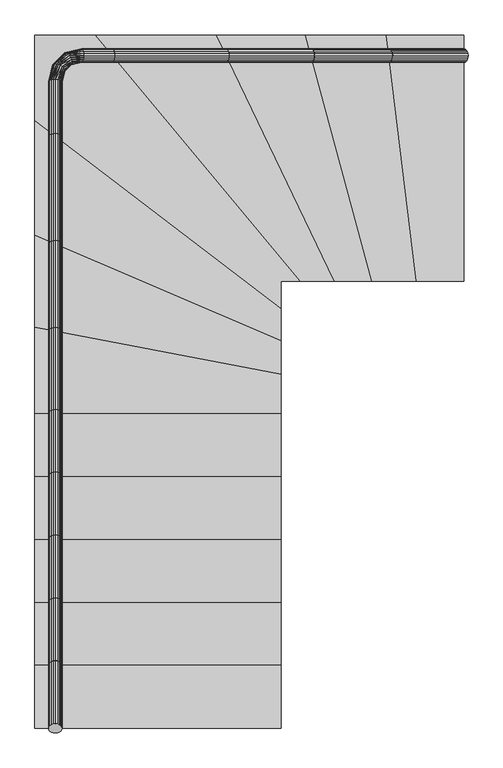
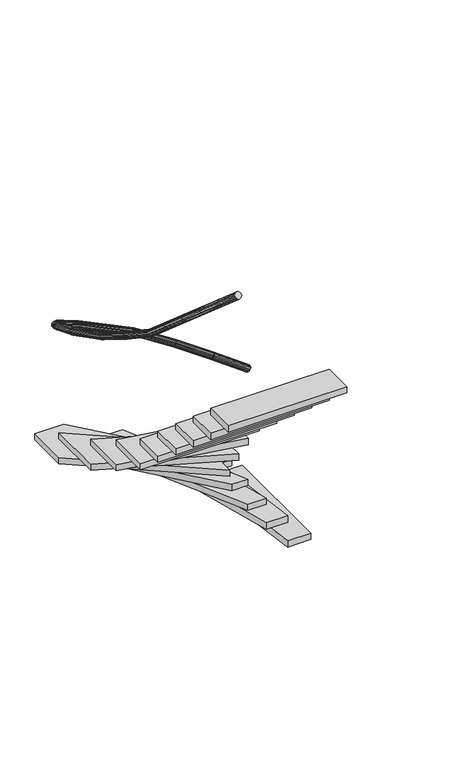
"""IFC4 building model written with IfcOpenShell, lengths in millimetres: stair geometry, 0_3d."""

from ifc_helpers import new_model, si_unit, frame, origin, origin_with_axes, place, context, project, spatial, polyline, outline, extrude, faceted_brep, source, transform, mapped, element, save


def stair_9af007b4(model_context):
    return source(origin(), model_context, "Body", "SolidModel", [
        extrude(outline(polyline([(1.2235871, -7.9923213), (0.0, 0.0), (1.2235871, 7.9923214), (4.7745751, 15.2022986), (10.3053687, 20.9241691), (17.2745751, 24.5978359), (25.0, 25.8636953), (32.7254249, 24.5978359), (39.6946313, 20.9241691), (45.2254249, 15.2022986), (48.7764129, 7.9923214), (50.0, 0.0), (48.7764129, -7.9923213), (45.2254249, -15.2022986), (39.6946313, -20.924169), (32.7254249, -24.5978359), (25.0, -25.8636953), (17.2745751, -24.5978359), (10.3053687, -20.924169), (4.7745751, -15.2022986), (1.2235871, -7.9923213)])), frame((50.0, 936.9712063, 2669.5592366), z_axis=(0.0, -0.7546055221634576, 0.6561787149248409), x_axis=(1.0, 0.0, 0.0)), (0.0, 0.0, 1.0), 304.7950131),
        extrude(outline(polyline([(970.0, 1651.5730429), (900.0, 1651.5730429), (900.0, 1551.5730429), (0.0, 2237.7659758), (0.0, 2551.5730429), (219.7566439, 2551.5730429), (970.0, 1651.5730429)])), frame((0.0, 0.0, 800.0), z_axis=(0.0, 0.0, 1.0), x_axis=(1.0, 0.0, 0.0)), (0.0, 0.0, 1.0), 50.0),
        extrude(outline(polyline([(1.2235871, -7.9923213), (0.0, 0.0), (1.2235871, 7.9923214), (4.7745751, 15.2022986), (10.3053687, 20.9241691), (17.2745751, 24.5978359), (25.0, 25.8636953), (32.7254249, 24.5978359), (39.6946313, 20.9241691), (45.2254249, 15.2022986), (48.7764129, 7.9923214), (50.0, 0.0), (48.7764129, -7.9923213), (45.2254249, -15.2022986), (39.6946313, -20.924169), (32.7254249, -24.5978359), (25.0, -25.8636953), (17.2745751, -24.5978359), (10.3053687, -20.924169), (4.7745751, -15.2022986), (1.2235871, -7.9923213)])), frame((50.0, 706.9712063, 2869.5592366), z_axis=(0.0, -0.7546055221634843, 0.6561787149248102), x_axis=(1.0, 0.0, 0.0)), (0.0, 0.0, 1.0), 304.7950131),
        extrude(outline(polyline([(1093.3486159, 1651.5730429), (970.0, 1651.5730429), (219.7566439, 2551.5730429), (662.4236343, 2551.5730429), (1093.3486159, 1651.5730429)])), frame((0.0, 0.0, 600.0), z_axis=(0.0, 0.0, 1.0), x_axis=(1.0, 0.0, 0.0)), (0.0, 0.0, 1.0), 50.0),
        faceted_brep([(51.2235871, 2177.2875031, 1862.2686626), (50.0, 2180.5832314, 1869.5592366), (51.2235871, 2183.8789598, 1876.8498106), (54.7745751, 2186.8520793, 1883.4267324), (60.3053687, 2189.2115603, 1888.6462072), (67.2745751, 2190.7264404, 1891.9973162), (75.0, 2191.2484324, 1893.1520297), (82.7254249, 2190.7264404, 1891.9973162), (89.6946313, 2189.2115603, 1888.6462072), (95.2254249, 2186.8520793, 1883.4267324), (98.7764129, 2183.8789598, 1876.8498106), (100.0, 2180.5832314, 1869.5592366), (98.7764129, 2177.2875031, 1862.2686626), (95.2254249, 2174.3143835, 1855.6917408), (89.6946313, 2171.9549025, 1850.4722661), (82.7254249, 2170.4400225, 1847.121157), (75.0, 2169.9180304, 1845.9664435), (67.2745751, 2170.4400225, 1847.121157), (60.3053687, 2171.9549025, 1850.4722661), (54.7745751, 2174.3143835, 1855.6917408), (51.2235871, 1791.6314427, 2076.5199053), (50.0, 1787.6876226, 2069.5592366), (51.2235871, 1783.7438024, 2062.5985679), (54.7745751, 1780.1860309, 2056.319258), (60.3053687, 1777.3625674, 2051.3359694), (67.2745751, 1775.5497922, 2048.1365012), (75.0, 1774.9251525, 2047.0340396), (82.7254249, 1775.5497922, 2048.1365012), (89.6946313, 1777.3625674, 2051.3359694), (95.2254249, 1780.1860309, 2056.319258), (98.7764129, 1783.7438024, 2062.5985679), (100.0, 1787.6876226, 2069.5592366), (98.7764129, 1791.6314427, 2076.5199053), (95.2254249, 1795.1892143, 2082.7992152), (89.6946313, 1798.0126778, 2087.7825038), (82.7254249, 1799.8254529, 2090.981972), (75.0, 1800.4500927, 2092.0844336), (67.2745751, 1799.8254529, 2090.981972), (60.3053687, 1798.0126778, 2087.7825038), (54.7745751, 1795.1892143, 2082.7992152)], [[[0, 1, 2, 3, 4, 5, 6, 7, 8, 9, 10, 11, 12, 13, 14, 15, 16, 17, 18, 19]], [[20, 21, 22, 23, 24, 25, 26, 27, 28, 29, 30, 31, 32, 33, 34, 35, 36, 37, 38, 39]], [[2, 1, 21, 20]], [[3, 2, 20, 39]], [[4, 3, 39, 38]], [[5, 4, 38, 37]], [[6, 5, 37, 36]], [[7, 6, 36, 35]], [[8, 7, 35, 34]], [[9, 8, 34, 33]], [[10, 9, 33, 32]], [[11, 10, 32, 31]], [[12, 11, 31, 30]], [[13, 12, 30, 29]], [[14, 13, 29, 28]], [[15, 14, 28, 27]], [[16, 15, 27, 26]], [[17, 16, 26, 25]], [[18, 17, 25, 24]], [[19, 18, 24, 23]], [[0, 19, 23, 22]], [[1, 0, 22, 21]]]),
        faceted_brep([(279.0658693, 2500.3494558, 1662.2350128), (282.2769235, 2501.5730429, 1669.5592366), (285.4879778, 2500.3494558, 1676.8834604), (288.3847117, 2496.7984678, 1683.4907382), (290.6835727, 2491.2676742, 1688.7343035), (292.1595323, 2484.2984678, 1692.1008796), (292.6681133, 2476.5730429, 1693.2609227), (292.1595323, 2468.8476181, 1692.1008796), (290.6835727, 2461.8784116, 1688.7343035), (288.3847117, 2456.3476181, 1683.4907382), (285.4879778, 2452.79663, 1676.8834604), (282.2769235, 2451.5730429, 1669.5592366), (279.0658693, 2452.79663, 1662.2350128), (276.1691354, 2456.3476181, 1655.627735), (273.8702744, 2461.8784116, 1650.3841697), (272.3943148, 2468.8476181, 1647.0175936), (271.8857337, 2476.5730429, 1645.8575505), (272.3943148, 2484.2984678, 1647.0175936), (273.8702744, 2491.2676742, 1650.3841697), (276.1691354, 2496.7984678, 1655.627735), (51.2235871, 2183.8789598, 1876.8498106), (50.0, 2180.5832314, 1869.5592366), (51.2235871, 2177.2875031, 1862.2686626), (54.7745751, 2174.3143835, 1855.6917408), (60.3053687, 2171.9549025, 1850.4722661), (67.2745751, 2170.4400225, 1847.121157), (75.0, 2169.9180304, 1845.9664435), (82.7254249, 2170.4400225, 1847.121157), (89.6946313, 2171.9549025, 1850.4722661), (95.2254249, 2174.3143835, 1855.6917408), (98.7764129, 2177.2875031, 1862.2686626), (100.0, 2180.5832314, 1869.5592366), (98.7764129, 2183.8789598, 1876.8498106), (95.2254249, 2186.8520793, 1883.4267324), (89.6946313, 2189.2115603, 1888.6462072), (82.7254249, 2190.7264404, 1891.9973162), (75.0, 2191.2484324, 1893.1520297), (67.2745751, 2190.7264404, 1891.9973162), (60.3053687, 2189.2115603, 1888.6462072), (54.7745751, 2186.8520793, 1883.4267324), (171.1411888, 2501.5730429, 1713.724975), (174.0928304, 2500.3494558, 1721.1522903), (176.7555448, 2496.7984678, 1727.8525682), (178.8686869, 2491.2676742, 1733.1699389), (180.2254077, 2484.2984678, 1736.583901), (180.6929018, 2476.5730429, 1737.7602722), (180.2254077, 2468.8476181, 1736.583901), (178.8686869, 2461.8784116, 1733.1699389), (176.7555448, 2456.3476181, 1727.8525682), (174.0928304, 2452.79663, 1721.1522903), (171.1411888, 2451.5730429, 1713.724975), (168.1895471, 2452.79663, 1706.2976597), (165.5268327, 2456.3476181, 1699.5973818), (163.4136906, 2461.8784116, 1694.2800111), (162.0569698, 2468.8476181, 1690.866049), (161.5894757, 2476.5730429, 1689.6896778), (162.0569698, 2484.2984678, 1690.866049), (163.4136906, 2491.2676742, 1694.2800111), (165.5268327, 2496.7984678, 1699.5973818), (168.1895471, 2500.3494558, 1706.2976597), (108.4388924, 2486.457503, 1738.6559048), (112.3547346, 2487.2072116, 1745.6899991), (117.06286, 2485.7372245, 1752.0355473), (122.1024044, 2482.1914344, 1757.0714029), (126.9800623, 2476.9169277, 1760.3046212), (131.2183743, 2470.43001, 1761.4187123), (134.4024651, 2463.365666, 1760.3046212), (136.2206536, 2456.4154029, 1757.0714029), (136.4949629, 2450.2595609, 1752.0355473), (135.1985416, 2445.5007167, 1745.6899991), (132.4582926, 2442.604699, 1738.6559048), (128.5424504, 2441.8549904, 1731.6218104), (123.834325, 2443.3249774, 1725.2762623), (118.7947805, 2446.8707676, 1720.2404067), (113.9171227, 2452.1452743, 1717.0071884), (109.6788106, 2458.632192, 1715.8930973), (106.4947198, 2465.696536, 1717.0071884), (104.6765313, 2472.6467991, 1720.2404067), (104.402222, 2478.8026411, 1725.2762623), (105.6986433, 2483.5614853, 1731.6218104), (65.11554, 2443.1341506, 1765.2077495), (68.0115576, 2445.8743996, 1772.2418439), (72.7704018, 2447.1708209, 1778.5873921), (78.9262439, 2446.8965116, 1783.6232476), (85.876507, 2445.0783231, 1786.8564659), (92.940851, 2441.8942323, 1787.970557), (99.4277686, 2437.6559202, 1786.8564659), (104.7022753, 2432.7782624, 1783.6232476), (108.2480655, 2427.7387179, 1778.5873921), (109.7180525, 2423.0305925, 1772.2418439), (108.9683439, 2419.1147504, 1765.2077495), (106.0723263, 2416.3745013, 1758.1736552), (101.313482, 2415.07808, 1751.828107), (95.15764, 2415.3523893, 1746.7922515), (88.2073769, 2417.1705778, 1743.5590332), (81.1430329, 2420.3546686, 1742.4449421), (74.6561152, 2424.5929807, 1743.5590332), (69.3816086, 2429.4706385, 1746.7922515), (65.8358184, 2434.510183, 1751.828107), (64.3658313, 2439.2183084, 1758.1736552), (50.0, 2380.4318542, 1790.1386793), (51.2235871, 2383.3834958, 1797.5659946), (54.7745751, 2386.0462102, 1804.2662726), (60.3053687, 2388.1593524, 1809.5836432), (67.2745751, 2389.5160731, 1812.9976054), (75.0, 2389.9835672, 1814.1739765), (82.7254249, 2389.5160731, 1812.9976054), (89.6946313, 2388.1593524, 1809.5836432), (95.2254249, 2386.0462102, 1804.2662726), (98.7764129, 2383.3834958, 1797.5659946), (100.0, 2380.4318542, 1790.1386793), (98.7764129, 2377.4802125, 1782.711364), (95.2254249, 2374.8174981, 1776.0110861), (89.6946313, 2372.704356, 1770.6937155), (82.7254249, 2371.3476352, 1767.2797533), (75.0, 2370.8801411, 1766.1033822), (67.2745751, 2371.3476352, 1767.2797533), (60.3053687, 2372.704356, 1770.6937155), (54.7745751, 2374.8174981, 1776.0110861), (51.2235871, 2377.4802125, 1782.711364)], [[[0, 1, 2, 3, 4, 5, 6, 7, 8, 9, 10, 11, 12, 13, 14, 15, 16, 17, 18, 19]], [[20, 21, 22, 23, 24, 25, 26, 27, 28, 29, 30, 31, 32, 33, 34, 35, 36, 37, 38, 39]], [[2, 1, 40, 41]], [[3, 2, 41, 42]], [[4, 3, 42, 43]], [[5, 4, 43, 44]], [[6, 5, 44, 45]], [[7, 6, 45, 46]], [[8, 7, 46, 47]], [[9, 8, 47, 48]], [[10, 9, 48, 49]], [[11, 10, 49, 50]], [[12, 11, 50, 51]], [[13, 12, 51, 52]], [[14, 13, 52, 53]], [[15, 14, 53, 54]], [[16, 15, 54, 55]], [[17, 16, 55, 56]], [[18, 17, 56, 57]], [[19, 18, 57, 58]], [[0, 19, 58, 59]], [[1, 0, 59, 40]], [[41, 40, 60]], [[61, 41, 60]], [[42, 41, 61]], [[62, 42, 61]], [[43, 42, 62]], [[63, 43, 62]], [[44, 43, 63]], [[64, 44, 63]], [[45, 44, 64]], [[65, 45, 64]], [[46, 45, 65]], [[66, 46, 65]], [[47, 46, 66]], [[67, 47, 66]], [[48, 47, 67]], [[68, 48, 67]], [[49, 48, 68]], [[69, 49, 68]], [[50, 49, 69]], [[70, 50, 69]], [[51, 50, 70]], [[71, 51, 70]], [[52, 51, 71]], [[72, 52, 71]], [[53, 52, 72]], [[73, 53, 72]], [[54, 53, 73]], [[74, 54, 73]], [[55, 54, 74]], [[75, 55, 74]], [[56, 55, 75]], [[76, 56, 75]], [[57, 56, 76]], [[77, 57, 76]], [[58, 57, 77]], [[78, 58, 77]], [[59, 58, 78]], [[79, 59, 78]], [[40, 59, 79]], [[60, 40, 79]], [[61, 60, 80]], [[81, 61, 80]], [[62, 61, 81]], [[82, 62, 81]], [[63, 62, 82]], [[83, 63, 82]], [[64, 63, 83]], [[84, 64, 83]], [[65, 64, 84]], [[85, 65, 84]], [[66, 65, 85]], [[86, 66, 85]], [[67, 66, 86]], [[87, 67, 86]], [[68, 67, 87]], [[88, 68, 87]], [[69, 68, 88]], [[89, 69, 88]], [[70, 69, 89]], [[90, 70, 89]], [[71, 70, 90]], [[91, 71, 90]], [[72, 71, 91]], [[92, 72, 91]], [[73, 72, 92]], [[93, 73, 92]], [[74, 73, 93]], [[94, 74, 93]], [[75, 74, 94]], [[95, 75, 94]], [[76, 75, 95]], [[96, 76, 95]], [[77, 76, 96]], [[97, 77, 96]], [[78, 77, 97]], [[98, 78, 97]], [[79, 78, 98]], [[99, 79, 98]], [[60, 79, 99]], [[80, 60, 99]], [[81, 80, 100]], [[101, 81, 100]], [[82, 81, 101]], [[102, 82, 101]], [[83, 82, 102]], [[103, 83, 102]], [[84, 83, 103]], [[104, 84, 103]], [[85, 84, 104]], [[105, 85, 104]], [[86, 85, 105]], [[106, 86, 105]], [[87, 86, 106]], [[107, 87, 106]], [[88, 87, 107]], [[108, 88, 107]], [[89, 88, 108]], [[109, 89, 108]], [[90, 89, 109]], [[110, 90, 109]], [[91, 90, 110]], [[111, 91, 110]], [[92, 91, 111]], [[112, 92, 111]], [[93, 92, 112]], [[113, 93, 112]], [[94, 93, 113]], [[114, 94, 113]], [[95, 94, 114]], [[115, 95, 114]], [[96, 95, 115]], [[116, 96, 115]], [[97, 96, 116]], [[117, 97, 116]], [[98, 97, 117]], [[118, 98, 117]], [[99, 98, 118]], [[119, 99, 118]], [[80, 99, 119]], [[100, 80, 119]], [[101, 100, 21, 20]], [[102, 101, 20, 39]], [[103, 102, 39, 38]], [[104, 103, 38, 37]], [[105, 104, 37, 36]], [[106, 105, 36, 35]], [[107, 106, 35, 34]], [[108, 107, 34, 33]], [[109, 108, 33, 32]], [[110, 109, 32, 31]], [[111, 110, 31, 30]], [[112, 111, 30, 29]], [[113, 112, 29, 28]], [[114, 113, 28, 27]], [[115, 114, 27, 26]], [[116, 115, 26, 25]], [[117, 116, 25, 24]], [[118, 117, 24, 23]], [[119, 118, 23, 22]], [[100, 119, 22, 21]]]),
        faceted_brep([(51.2235871, 1162.120888, 2463.1855148), (50.0, 1166.9712063, 2469.5592366), (51.2235871, 1171.8215247, 2475.9329585), (54.7745751, 1176.1970601, 2481.682776), (60.3053687, 1179.6695046, 2486.2458571), (67.2745751, 1181.8989513, 2489.1755354), (75.0, 1182.6671663, 2490.1850338), (82.7254249, 1181.8989513, 2489.1755354), (89.6946313, 1179.6695046, 2486.2458571), (95.2254249, 1176.1970601, 2481.682776), (98.7764129, 1171.8215247, 2475.9329585), (100.0, 1166.9712063, 2469.5592366), (98.7764129, 1162.120888, 2463.1855148), (95.2254249, 1157.7453526, 2457.4356972), (89.6946313, 1154.272908, 2452.8726162), (82.7254249, 1152.0434614, 2449.9429378), (75.0, 1151.2752464, 2448.9334394), (67.2745751, 1152.0434614, 2449.9429378), (60.3053687, 1154.272908, 2452.8726162), (54.7745751, 1157.7453526, 2457.4356972), (51.2235871, 942.2155975, 2675.5902865), (50.0, 936.9712063, 2669.5592366), (51.2235871, 931.7268152, 2663.5281868), (54.7745751, 926.9957815, 2658.0874981), (60.3053687, 923.241212, 2653.7697431), (67.2745751, 920.83063, 2650.9975738), (75.0, 920.0, 2650.0423493), (82.7254249, 920.83063, 2650.9975738), (89.6946313, 923.241212, 2653.7697431), (95.2254249, 926.9957815, 2658.0874981), (98.7764129, 931.7268152, 2663.5281868), (100.0, 936.9712063, 2669.5592366), (98.7764129, 942.2155975, 2675.5902865), (95.2254249, 946.9466311, 2681.0309751), (89.6946313, 950.7012007, 2685.3487301), (82.7254249, 953.1117827, 2688.1208994), (75.0, 953.9424127, 2689.0761239), (67.2745751, 953.1117827, 2688.1208994), (60.3053687, 950.7012007, 2685.3487301), (54.7745751, 946.9466311, 2681.0309751)], [[[0, 1, 2, 3, 4, 5, 6, 7, 8, 9, 10, 11, 12, 13, 14, 15, 16, 17, 18, 19]], [[20, 21, 22, 23, 24, 25, 26, 27, 28, 29, 30, 31, 32, 33, 34, 35, 36, 37, 38, 39]], [[2, 1, 21, 20]], [[3, 2, 20, 39]], [[4, 3, 39, 38]], [[5, 4, 38, 37]], [[6, 5, 37, 36]], [[7, 6, 36, 35]], [[8, 7, 35, 34]], [[9, 8, 34, 33]], [[10, 9, 33, 32]], [[11, 10, 32, 31]], [[12, 11, 31, 30]], [[13, 12, 30, 29]], [[14, 13, 29, 28]], [[15, 14, 28, 27]], [[16, 15, 27, 26]], [[17, 16, 26, 25]], [[18, 17, 25, 24]], [[19, 18, 24, 23]], [[0, 19, 23, 22]], [[1, 0, 22, 21]]]),
        extrude(outline(polyline([(900.0, 936.9712063), (900.0, 706.9712063), (0.0, 706.9712063), (0.0, 936.9712063), (900.0, 936.9712063)])), frame((0.0, 0.0, 1800.0), z_axis=(0.0, 0.0, 1.0), x_axis=(1.0, 0.0, 0.0)), (0.0, 0.0, 1.0), 50.0),
        extrude(outline(polyline([(900.0, 1310.8135078), (900.0, 1166.9712063), (0.0, 1166.9712063), (0.0, 1483.1289049), (900.0, 1310.8135078)])), frame((0.0, 0.0, 1400.0), z_axis=(0.0, 0.0, 1.0), x_axis=(1.0, 0.0, 0.0)), (0.0, 0.0, 1.0), 50.0),
        extrude(outline(polyline([(900.0, 1434.6945611), (900.0, 1310.8135078), (0.0, 1483.1289049), (0.0, 1819.7779009), (900.0, 1434.6945611)])), frame((0.0, 0.0, 1200.0), z_axis=(0.0, 0.0, 1.0), x_axis=(1.0, 0.0, 0.0)), (0.0, 0.0, 1.0), 50.0),
        faceted_brep([(1565.3069331, 2500.3494558, 863.0898994), (1570.0, 2501.5730429, 869.5592366), (1574.6930669, 2500.3494558, 876.0285738), (1578.9267437, 2496.7984678, 881.8646473), (1582.2866086, 2491.2676742, 886.4961814), (1584.4437746, 2484.2984678, 889.4698093), (1585.1870834, 2476.5730429, 890.4944517), (1584.4437746, 2468.8476181, 889.4698093), (1582.2866086, 2461.8784116, 886.4961814), (1578.9267437, 2456.3476181, 881.8646473), (1574.6930669, 2452.79663, 876.0285738), (1570.0, 2451.5730429, 869.5592366), (1565.3069331, 2452.79663, 863.0898994), (1561.0732563, 2456.3476181, 857.2538259), (1557.7133914, 2461.8784116, 852.6222918), (1555.5562254, 2468.8476181, 849.6486639), (1554.8129166, 2476.5730429, 848.6240215), (1555.5562254, 2484.2984678, 849.6486639), (1557.7133914, 2491.2676742, 852.6222918), (1561.0732563, 2496.7984678, 857.2538259), (1298.9424936, 2500.3494558, 1076.0669753), (1294.3023627, 2501.5730429, 1069.5592366), (1289.6622317, 2500.3494558, 1063.0514979), (1285.4763091, 2496.7984678, 1057.1807821), (1282.1543421, 2491.2676742, 1052.5217556), (1280.021508, 2484.2984678, 1049.5304765), (1279.2865835, 2476.5730429, 1048.4997519), (1280.021508, 2468.8476181, 1049.5304765), (1282.1543421, 2461.8784116, 1052.5217556), (1285.4763091, 2456.3476181, 1057.1807821), (1289.6622317, 2452.79663, 1063.0514979), (1294.3023627, 2451.5730429, 1069.5592366), (1298.9424936, 2452.79663, 1076.0669753), (1303.1284163, 2456.3476181, 1081.9376911), (1306.4503833, 2461.8784116, 1086.5967176), (1308.5832174, 2468.8476181, 1089.5879968), (1309.3181419, 2476.5730429, 1090.6187213), (1308.5832174, 2484.2984678, 1089.5879968), (1306.4503833, 2491.2676742, 1086.5967176), (1303.1284163, 2496.7984678, 1081.9376911)], [[[0, 1, 2, 3, 4, 5, 6, 7, 8, 9, 10, 11, 12, 13, 14, 15, 16, 17, 18, 19]], [[20, 21, 22, 23, 24, 25, 26, 27, 28, 29, 30, 31, 32, 33, 34, 35, 36, 37, 38, 39]], [[2, 1, 21, 20]], [[3, 2, 20, 39]], [[4, 3, 39, 38]], [[5, 4, 38, 37]], [[6, 5, 37, 36]], [[7, 6, 36, 35]], [[8, 7, 35, 34]], [[9, 8, 34, 33]], [[10, 9, 33, 32]], [[11, 10, 32, 31]], [[12, 11, 31, 30]], [[13, 12, 30, 29]], [[14, 13, 29, 28]], [[15, 14, 28, 27]], [[16, 15, 27, 26]], [[17, 16, 26, 25]], [[18, 17, 25, 24]], [[19, 18, 24, 23]], [[0, 19, 23, 22]], [[1, 0, 22, 21]]]),
        extrude(outline(polyline([(1.2235871, -7.9923213), (0.0, 0.0), (1.2235871, 7.9923214), (4.7745751, 15.2022986), (10.3053687, 20.9241691), (17.2745751, 24.5978359), (25.0, 25.8636953), (32.7254249, 24.5978359), (39.6946313, 20.9241691), (45.2254249, 15.2022986), (48.7764129, 7.9923214), (50.0, 0.0), (48.7764129, -7.9923213), (45.2254249, -15.2022986), (39.6946313, -20.924169), (32.7254249, -24.5978359), (25.0, -25.8636953), (17.2745751, -24.5978359), (10.3053687, -20.924169), (4.7745751, -15.2022986), (1.2235871, -7.9923213)])), frame((50.0, 476.9712063, 3069.5592366), z_axis=(0.0, -0.754605522163458, 0.6561787149248404), x_axis=(1.0, 0.0, 0.0)), (0.0, 0.0, 1.0), 304.7950131),
        faceted_brep([(51.2235871, 1464.4379829, 2262.8415677), (50.0, 1468.7692885, 2269.5592366), (51.2235871, 1473.100594, 2276.2769055), (54.7745751, 1477.0079212, 2282.3370022), (60.3053687, 1480.1087936, 2287.1463221), (67.2745751, 1482.0996763, 2290.2340956), (75.0, 1482.7856877, 2291.2980698), (82.7254249, 1482.0996763, 2290.2340956), (89.6946313, 1480.1087936, 2287.1463221), (95.2254249, 1477.0079212, 2282.3370022), (98.7764129, 1473.100594, 2276.2769055), (100.0, 1468.7692885, 2269.5592366), (98.7764129, 1464.4379829, 2262.8415677), (95.2254249, 1460.5306557, 2256.781471), (89.6946313, 1457.4297833, 2251.9721511), (82.7254249, 1455.4389007, 2248.8843776), (75.0, 1454.7528893, 2247.8204034), (67.2745751, 1455.4389007, 2248.8843776), (60.3053687, 1457.4297833, 2251.9721511), (54.7745751, 1460.5306557, 2256.781471), (51.2235871, 1171.8215247, 2475.9329585), (50.0, 1166.9712063, 2469.5592366), (51.2235871, 1162.120888, 2463.1855148), (54.7745751, 1157.7453526, 2457.4356972), (60.3053687, 1154.272908, 2452.8726162), (67.2745751, 1152.0434614, 2449.9429378), (75.0, 1151.2752464, 2448.9334394), (82.7254249, 1152.0434614, 2449.9429378), (89.6946313, 1154.272908, 2452.8726162), (95.2254249, 1157.7453526, 2457.4356972), (98.7764129, 1162.120888, 2463.1855148), (100.0, 1166.9712063, 2469.5592366), (98.7764129, 1171.8215247, 2475.9329585), (95.2254249, 1176.1970601, 2481.682776), (89.6946313, 1179.6695046, 2486.2458571), (82.7254249, 1181.8989513, 2489.1755354), (75.0, 1182.6671663, 2490.1850338), (67.2745751, 1181.8989513, 2489.1755354), (60.3053687, 1179.6695046, 2486.2458571), (54.7745751, 1176.1970601, 2481.682776)], [[[0, 1, 2, 3, 4, 5, 6, 7, 8, 9, 10, 11, 12, 13, 14, 15, 16, 17, 18, 19]], [[20, 21, 22, 23, 24, 25, 26, 27, 28, 29, 30, 31, 32, 33, 34, 35, 36, 37, 38, 39]], [[2, 1, 21, 20]], [[3, 2, 20, 39]], [[4, 3, 39, 38]], [[5, 4, 38, 37]], [[6, 5, 37, 36]], [[7, 6, 36, 35]], [[8, 7, 35, 34]], [[9, 8, 34, 33]], [[10, 9, 33, 32]], [[11, 10, 32, 31]], [[12, 11, 31, 30]], [[13, 12, 30, 29]], [[14, 13, 29, 28]], [[15, 14, 28, 27]], [[16, 15, 27, 26]], [[17, 16, 26, 25]], [[18, 17, 25, 24]], [[19, 18, 24, 23]], [[0, 19, 23, 22]], [[1, 0, 22, 21]]]),
        extrude(outline(polyline([(900.0, 1551.5730429), (900.0, 1434.6945611), (0.0, 1819.7779009), (0.0, 2237.7659758), (900.0, 1551.5730429)])), frame((0.0, 0.0, 1000.0), z_axis=(0.0, 0.0, 1.0), x_axis=(1.0, 0.0, 0.0)), (0.0, 0.0, 1.0), 50.0),
        extrude(outline(polyline([(1231.3290941, 1651.5730429), (1093.3486159, 1651.5730429), (662.4236343, 2551.5730429), (988.6709059, 2551.5730429), (1231.3290941, 1651.5730429)])), frame((0.0, 0.0, 400.0), z_axis=(0.0, 0.0, 1.0), x_axis=(1.0, 0.0, 0.0)), (0.0, 0.0, 1.0), 50.0),
        faceted_brep([(694.4240305, 2500.3494558, 1462.5710073), (698.3340494, 2501.5730429, 1469.5592366), (702.2440682, 2500.3494558, 1476.5474659), (705.7713472, 2496.7984678, 1482.8516386), (708.5706116, 2491.2676742, 1487.8546583), (710.36785, 2484.2984678, 1491.0667948), (710.9871362, 2476.5730429, 1492.1736216), (710.36785, 2468.8476181, 1491.0667948), (708.5706116, 2461.8784116, 1487.8546583), (705.7713472, 2456.3476181, 1482.8516386), (702.2440682, 2452.79663, 1476.5474659), (698.3340494, 2451.5730429, 1469.5592366), (694.4240305, 2452.79663, 1462.5710073), (690.8967516, 2456.3476181, 1456.2668346), (688.0974871, 2461.8784116, 1451.2638149), (686.3002487, 2468.8476181, 1448.0516784), (685.6809626, 2476.5730429, 1446.9448517), (686.3002487, 2484.2984678, 1448.0516784), (688.0974871, 2491.2676742, 1451.2638149), (690.8967516, 2496.7984678, 1456.2668346), (285.4879778, 2500.3494558, 1676.8834604), (282.2769235, 2501.5730429, 1669.5592366), (279.0658693, 2500.3494558, 1662.2350128), (276.1691354, 2496.7984678, 1655.627735), (273.8702744, 2491.2676742, 1650.3841697), (272.3943148, 2484.2984678, 1647.0175936), (271.8857337, 2476.5730429, 1645.8575505), (272.3943148, 2468.8476181, 1647.0175936), (273.8702744, 2461.8784116, 1650.3841697), (276.1691354, 2456.3476181, 1655.627735), (279.0658693, 2452.79663, 1662.2350128), (282.2769235, 2451.5730429, 1669.5592366), (285.4879778, 2452.79663, 1676.8834604), (288.3847117, 2456.3476181, 1683.4907382), (290.6835727, 2461.8784116, 1688.7343035), (292.1595323, 2468.8476181, 1692.1008796), (292.6681133, 2476.5730429, 1693.2609227), (292.1595323, 2484.2984678, 1692.1008796), (290.6835727, 2491.2676742, 1688.7343035), (288.3847117, 2496.7984678, 1683.4907382)], [[[0, 1, 2, 3, 4, 5, 6, 7, 8, 9, 10, 11, 12, 13, 14, 15, 16, 17, 18, 19]], [[20, 21, 22, 23, 24, 25, 26, 27, 28, 29, 30, 31, 32, 33, 34, 35, 36, 37, 38, 39]], [[2, 1, 21, 20]], [[3, 2, 20, 39]], [[4, 3, 39, 38]], [[5, 4, 38, 37]], [[6, 5, 37, 36]], [[7, 6, 36, 35]], [[8, 7, 35, 34]], [[9, 8, 34, 33]], [[10, 9, 33, 32]], [[11, 10, 32, 31]], [[12, 11, 31, 30]], [[13, 12, 30, 29]], [[14, 13, 29, 28]], [[15, 14, 28, 27]], [[16, 15, 27, 26]], [[17, 16, 26, 25]], [[18, 17, 25, 24]], [[19, 18, 24, 23]], [[0, 19, 23, 22]], [[1, 0, 22, 21]]]),
        extrude(outline(polyline([(900.0, 1166.9712063), (900.0, 936.9712063), (0.0, 936.9712063), (0.0, 1166.9712063), (900.0, 1166.9712063)])), frame((0.0, 0.0, 1600.0), z_axis=(0.0, 0.0, 1.0), x_axis=(1.0, 0.0, 0.0)), (0.0, 0.0, 1.0), 50.0),
        faceted_brep([(1289.6622317, 2500.3494558, 1063.0514979), (1294.3023627, 2501.5730429, 1069.5592366), (1298.9424936, 2500.3494558, 1076.0669753), (1303.1284163, 2496.7984678, 1081.9376911), (1306.4503833, 2491.2676742, 1086.5967176), (1308.5832174, 2484.2984678, 1089.5879968), (1309.3181419, 2476.5730429, 1090.6187213), (1308.5832174, 2468.8476181, 1089.5879968), (1306.4503833, 2461.8784116, 1086.5967176), (1303.1284163, 2456.3476181, 1081.9376911), (1298.9424936, 2452.79663, 1076.0669753), (1294.3023627, 2451.5730429, 1069.5592366), (1289.6622317, 2452.79663, 1063.0514979), (1285.4763091, 2456.3476181, 1057.1807821), (1282.1543421, 2461.8784116, 1052.5217556), (1280.021508, 2468.8476181, 1049.5304765), (1279.2865835, 2476.5730429, 1048.4997519), (1280.021508, 2484.2984678, 1049.5304765), (1282.1543421, 2491.2676742, 1052.5217556), (1285.4763091, 2496.7984678, 1057.1807821), (1013.3510842, 2500.3494558, 1276.1941386), (1008.8924216, 2501.5730429, 1269.5592366), (1004.433759, 2500.3494558, 1262.9243346), (1000.4115414, 2496.7984678, 1256.9389031), (997.2194914, 2491.2676742, 1252.1888377), (995.1700692, 2484.2984678, 1249.139108), (994.4638864, 2476.5730429, 1248.0882427), (995.1700692, 2468.8476181, 1249.139108), (997.2194914, 2461.8784116, 1252.1888377), (1000.4115414, 2456.3476181, 1256.9389031), (1004.433759, 2452.79663, 1262.9243346), (1008.8924216, 2451.5730429, 1269.5592366), (1013.3510842, 2452.79663, 1276.1941386), (1017.3733018, 2456.3476181, 1282.1795702), (1020.5653518, 2461.8784116, 1286.9296355), (1022.614774, 2468.8476181, 1289.9793652), (1023.3209568, 2476.5730429, 1291.0302305), (1022.614774, 2484.2984678, 1289.9793652), (1020.5653518, 2491.2676742, 1286.9296355), (1017.3733018, 2496.7984678, 1282.1795702)], [[[0, 1, 2, 3, 4, 5, 6, 7, 8, 9, 10, 11, 12, 13, 14, 15, 16, 17, 18, 19]], [[20, 21, 22, 23, 24, 25, 26, 27, 28, 29, 30, 31, 32, 33, 34, 35, 36, 37, 38, 39]], [[2, 1, 21, 20]], [[3, 2, 20, 39]], [[4, 3, 39, 38]], [[5, 4, 38, 37]], [[6, 5, 37, 36]], [[7, 6, 36, 35]], [[8, 7, 35, 34]], [[9, 8, 34, 33]], [[10, 9, 33, 32]], [[11, 10, 32, 31]], [[12, 11, 31, 30]], [[13, 12, 30, 29]], [[14, 13, 29, 28]], [[15, 14, 28, 27]], [[16, 15, 27, 26]], [[17, 16, 26, 25]], [[18, 17, 25, 24]], [[19, 18, 24, 23]], [[0, 19, 23, 22]], [[1, 0, 22, 21]]]),
        faceted_brep([(51.2235871, 1783.7438024, 2062.5985679), (50.0, 1787.6876226, 2069.5592366), (51.2235871, 1791.6314427, 2076.5199053), (54.7745751, 1795.1892143, 2082.7992152), (60.3053687, 1798.0126778, 2087.7825038), (67.2745751, 1799.8254529, 2090.981972), (75.0, 1800.4500927, 2092.0844336), (82.7254249, 1799.8254529, 2090.981972), (89.6946313, 1798.0126778, 2087.7825038), (95.2254249, 1795.1892143, 2082.7992152), (98.7764129, 1791.6314427, 2076.5199053), (100.0, 1787.6876226, 2069.5592366), (98.7764129, 1783.7438024, 2062.5985679), (95.2254249, 1780.1860309, 2056.319258), (89.6946313, 1777.3625674, 2051.3359694), (82.7254249, 1775.5497922, 2048.1365012), (75.0, 1774.9251525, 2047.0340396), (67.2745751, 1775.5497922, 2048.1365012), (60.3053687, 1777.3625674, 2051.3359694), (54.7745751, 1780.1860309, 2056.319258), (51.2235871, 1473.100594, 2276.2769055), (50.0, 1468.7692885, 2269.5592366), (51.2235871, 1464.4379829, 2262.8415677), (54.7745751, 1460.5306557, 2256.781471), (60.3053687, 1457.4297833, 2251.9721511), (67.2745751, 1455.4389007, 2248.8843776), (75.0, 1454.7528893, 2247.8204034), (82.7254249, 1455.4389007, 2248.8843776), (89.6946313, 1457.4297833, 2251.9721511), (95.2254249, 1460.5306557, 2256.781471), (98.7764129, 1464.4379829, 2262.8415677), (100.0, 1468.7692885, 2269.5592366), (98.7764129, 1473.100594, 2276.2769055), (95.2254249, 1477.0079212, 2282.3370022), (89.6946313, 1480.1087936, 2287.1463221), (82.7254249, 1482.0996763, 2290.2340956), (75.0, 1482.7856877, 2291.2980698), (67.2745751, 1482.0996763, 2290.2340956), (60.3053687, 1480.1087936, 2287.1463221), (54.7745751, 1477.0079212, 2282.3370022)], [[[0, 1, 2, 3, 4, 5, 6, 7, 8, 9, 10, 11, 12, 13, 14, 15, 16, 17, 18, 19]], [[20, 21, 22, 23, 24, 25, 26, 27, 28, 29, 30, 31, 32, 33, 34, 35, 36, 37, 38, 39]], [[2, 1, 21, 20]], [[3, 2, 20, 39]], [[4, 3, 39, 38]], [[5, 4, 38, 37]], [[6, 5, 37, 36]], [[7, 6, 36, 35]], [[8, 7, 35, 34]], [[9, 8, 34, 33]], [[10, 9, 33, 32]], [[11, 10, 32, 31]], [[12, 11, 31, 30]], [[13, 12, 30, 29]], [[14, 13, 29, 28]], [[15, 14, 28, 27]], [[16, 15, 27, 26]], [[17, 16, 26, 25]], [[18, 17, 25, 24]], [[19, 18, 24, 23]], [[0, 19, 23, 22]], [[1, 0, 22, 21]]]),
        extrude(outline(polyline([(1394.8371648, 1651.5730429), (1231.3290941, 1651.5730429), (988.6709059, 2551.5730429), (1285.1628352, 2551.5730429), (1394.8371648, 1651.5730429)])), frame((0.0, 0.0, 200.0), z_axis=(0.0, 0.0, 1.0), x_axis=(1.0, 0.0, 0.0)), (0.0, 0.0, 1.0), 50.0),
        extrude(outline(polyline([(1570.0, 1651.5730429), (1394.8371648, 1651.5730429), (1285.1628352, 2551.5730429), (1570.0, 2551.5730429), (1570.0, 1651.5730429)])), origin_with_axes(), (0.0, 0.0, 1.0), 50.0),
        faceted_brep([(1004.433759, 2500.3494558, 1262.9243346), (1008.8924216, 2501.5730429, 1269.5592366), (1013.3510842, 2500.3494558, 1276.1941386), (1017.3733018, 2496.7984678, 1282.1795702), (1020.5653518, 2491.2676742, 1286.9296355), (1022.614774, 2484.2984678, 1289.9793652), (1023.3209568, 2476.5730429, 1291.0302305), (1022.614774, 2468.8476181, 1289.9793652), (1020.5653518, 2461.8784116, 1286.9296355), (1017.3733018, 2456.3476181, 1282.1795702), (1013.3510842, 2452.79663, 1276.1941386), (1008.8924216, 2451.5730429, 1269.5592366), (1004.433759, 2452.79663, 1262.9243346), (1000.4115414, 2456.3476181, 1256.9389031), (997.2194914, 2461.8784116, 1252.1888377), (995.1700692, 2468.8476181, 1249.139108), (994.4638864, 2476.5730429, 1248.0882427), (995.1700692, 2484.2984678, 1249.139108), (997.2194914, 2491.2676742, 1252.1888377), (1000.4115414, 2496.7984678, 1256.9389031), (702.2440682, 2500.3494558, 1476.5474659), (698.3340494, 2501.5730429, 1469.5592366), (694.4240305, 2500.3494558, 1462.5710073), (690.8967516, 2496.7984678, 1456.2668346), (688.0974871, 2491.2676742, 1451.2638149), (686.3002487, 2484.2984678, 1448.0516784), (685.6809626, 2476.5730429, 1446.9448517), (686.3002487, 2468.8476181, 1448.0516784), (688.0974871, 2461.8784116, 1451.2638149), (690.8967516, 2456.3476181, 1456.2668346), (694.4240305, 2452.79663, 1462.5710073), (698.3340494, 2451.5730429, 1469.5592366), (702.2440682, 2452.79663, 1476.5474659), (705.7713472, 2456.3476181, 1482.8516386), (708.5706116, 2461.8784116, 1487.8546583), (710.36785, 2468.8476181, 1491.0667948), (710.9871362, 2476.5730429, 1492.1736216), (710.36785, 2484.2984678, 1491.0667948), (708.5706116, 2491.2676742, 1487.8546583), (705.7713472, 2496.7984678, 1482.8516386)], [[[0, 1, 2, 3, 4, 5, 6, 7, 8, 9, 10, 11, 12, 13, 14, 15, 16, 17, 18, 19]], [[20, 21, 22, 23, 24, 25, 26, 27, 28, 29, 30, 31, 32, 33, 34, 35, 36, 37, 38, 39]], [[2, 1, 21, 20]], [[3, 2, 20, 39]], [[4, 3, 39, 38]], [[5, 4, 38, 37]], [[6, 5, 37, 36]], [[7, 6, 36, 35]], [[8, 7, 35, 34]], [[9, 8, 34, 33]], [[10, 9, 33, 32]], [[11, 10, 32, 31]], [[12, 11, 31, 30]], [[13, 12, 30, 29]], [[14, 13, 29, 28]], [[15, 14, 28, 27]], [[16, 15, 27, 26]], [[17, 16, 26, 25]], [[18, 17, 25, 24]], [[19, 18, 24, 23]], [[0, 19, 23, 22]], [[1, 0, 22, 21]]]),
        extrude(outline(polyline([(900.0, 706.9712063), (900.0, 476.9712063), (0.0, 476.9712063), (0.0, 706.9712063), (900.0, 706.9712063)])), frame((0.0, 0.0, 2000.0), z_axis=(0.0, 0.0, 1.0), x_axis=(1.0, 0.0, 0.0)), (0.0, 0.0, 1.0), 50.0),
        extrude(outline(polyline([(900.0, 476.9712063), (900.0, 246.9712063), (0.0, 246.9712063), (0.0, 476.9712063), (900.0, 476.9712063)])), frame((0.0, 0.0, 2200.0), z_axis=(0.0, 0.0, 1.0), x_axis=(1.0, 0.0, 0.0)), (0.0, 0.0, 1.0), 50.0),
        extrude(outline(polyline([(1.2235871, -7.9923213), (0.0, 0.0), (1.2235871, 7.9923214), (4.7745751, 15.2022986), (10.3053687, 20.9241691), (17.2745751, 24.5978359), (25.0, 25.8636953), (32.7254249, 24.5978359), (39.6946313, 20.9241691), (45.2254249, 15.2022986), (48.7764129, 7.9923214), (50.0, 0.0), (48.7764129, -7.9923213), (45.2254249, -15.2022986), (39.6946313, -20.924169), (32.7254249, -24.5978359), (25.0, -25.8636953), (17.2745751, -24.5978359), (10.3053687, -20.924169), (4.7745751, -15.2022986), (1.2235871, -7.9923213)])), frame((50.0, 246.9712063, 3269.5592366), z_axis=(0.0, -0.7546055221634859, 0.6561787149248085), x_axis=(1.0, 0.0, 0.0)), (0.0, 0.0, 1.0), 304.7950131),
        extrude(outline(polyline([(900.0, 246.9712063), (900.0, 16.9712063), (0.0, 16.9712063), (0.0, 246.9712063), (900.0, 246.9712063)])), frame((0.0, 0.0, 2400.0), z_axis=(0.0, 0.0, 1.0), x_axis=(1.0, 0.0, 0.0)), (0.0, 0.0, 1.0), 50.0),
    ])


if __name__ == "__main__":
    model = new_model("IFC4")
    model_context = context("Model", 3, world=origin())
    ifc_project = project(units=[si_unit("LENGTHUNIT", "METRE", prefix="MILLI")], contexts=[model_context])
    site = spatial("IfcSite", under=ifc_project)
    building = spatial("IfcBuilding", under=site)
    placement = place(None, origin())
    stair_shape = stair_9af007b4(model_context)
    element("IfcStair", 1, ObjectType="0_3d", at=placement, inside=building, context=model_context, shape_type="MappedRepresentation", body=[
        mapped(stair_shape, transform((0.0, 0.0, 0.0), x_axis=(1.0, 0.0, 0.0), y_axis=(0.0, 1.0, 0.0), z_axis=(0.0, 0.0, 1.0))),
    ])
    save(model, "model.ifc")

# Revit data of these elements
# Element 1 (IfcStair, "0_3d")
#   Materials on its faces: "*1", "weiss"
# Materials
#   "*1": class "Unassigned", colour RGB 175 175 175, transparency 0
#   "weiss": class "Unassigned", colour RGB 255 255 255, transparency 0
